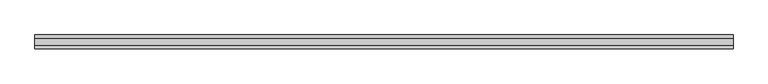
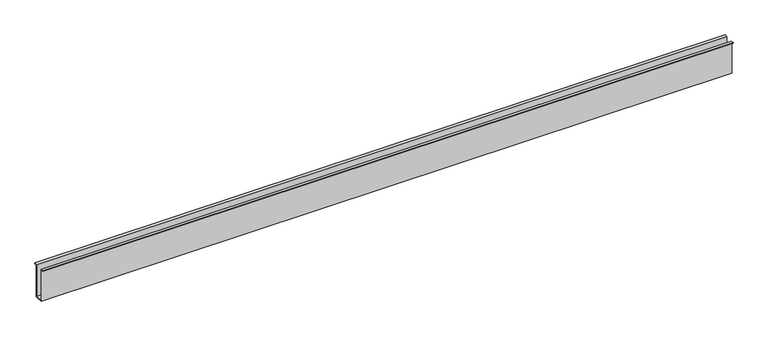
"""IFC4 building model written with IfcOpenShell, lengths in millimetres: railing geometry, ML_Perfil U de embutir2 : ML_Perfil U de embutir."""

from ifc_helpers import new_model, si_unit, frame, origin, place, context, project, spatial, polyline, outline, extrude, source, transform, mapped, element, save


def railing_c8eab29c(model_context):
    return source(origin(), model_context, "Body", "SweptSolid", [
        extrude(outline(polyline([(1832.4523952, 3702.0), (1832.4523952, 3594.0), (1856.4523952, 3594.0), (1856.4523952, 3702.0), (1866.9523952, 3702.0), (1866.9523952, 3700.0), (1858.4523952, 3700.0), (1858.4523952, 3592.0), (1830.4523952, 3592.0), (1830.4523952, 3700.0), (1821.9523952, 3700.0), (1821.9523952, 3702.0), (1832.4523952, 3702.0)])), frame((-12226.1487231, 0.0, 0.0), z_axis=(1.0, 0.0, 0.0), x_axis=(0.0, 1.0, 0.0)), (0.0, 0.0, 1.0), 2240.0),
    ])


if __name__ == "__main__":
    model = new_model("IFC4")
    model_context = context("Model", 3, world=origin())
    ifc_project = project(units=[si_unit("LENGTHUNIT", "METRE", prefix="MILLI")], contexts=[model_context])
    site = spatial("IfcSite", under=ifc_project)
    building = spatial("IfcBuilding", under=site)
    placement = place(None, origin())
    railing_shape = railing_c8eab29c(model_context)
    element("IfcRailing", 1, ObjectType="ML_Perfil U de embutir2 : ML_Perfil U de embutir", at=placement, inside=building, context=model_context, shape_type="MappedRepresentation", body=[
        mapped(railing_shape, transform((0.0, 0.0, 0.0), x_axis=(1.0, 0.0, 0.0), y_axis=(0.0, 1.0, 0.0), z_axis=(0.0, 0.0, 1.0))),
    ])
    save(model, "model.ifc")

# Revit data of these elements
# Type "ML_Perfil U de embutir2 : ML_Perfil U de embutir"
#   ME_Compr [instance default] = 2.24 m
#   ME_Material Perfil [instance default] = .ALUMÍNIO COM PINTURA ELETROSTÁTICA BRANCA
# Element 1 (IfcRailing, "ML_Perfil U de embutir2 : ML_Perfil U de embutir")
#   Materials on its faces: ".ALUMÍNIO COM PINTURA ELETROSTÁTICA BRANCA"
# Materials
#   ".ALUMÍNIO COM PINTURA ELETROSTÁTICA BRANCA": class "CC_METAIS", colour RGB 241 241 241, transparency 0, Cost = 0
